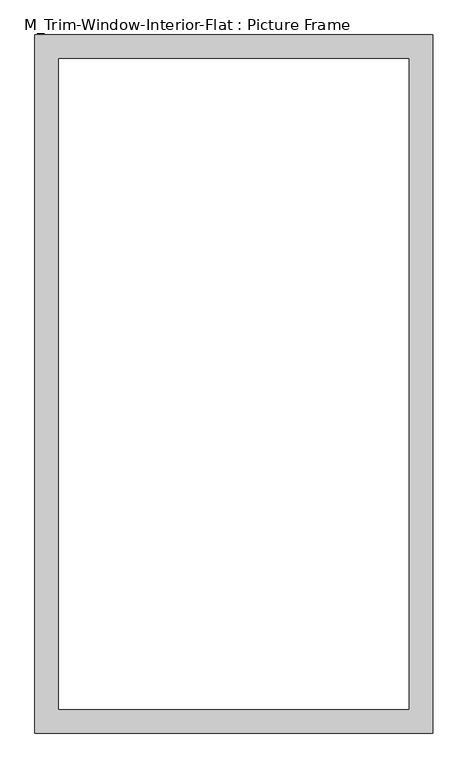
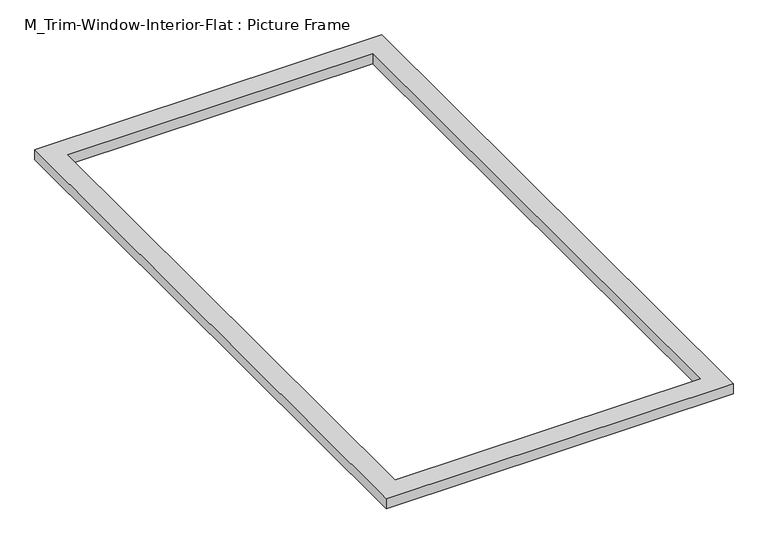
"""IFC4 building model written with IfcOpenShell, lengths in millimetres: proxy geometry, M_Trim-Window-Interior-Flat : Picture Frame."""

import ifcopenshell
import ifcopenshell.guid

model = None  # the IFC model being written
_history = None  # IfcOwnerHistory: only IFC2X3 demands one
_inside = {}  # id of a spatial element -> (the spatial element, [elements in it])
_under = {}  # id of a project, library or spatial element -> (it, [spatial elements below it])
_declared = {}  # id of a project -> (the project, [libraries it declares])
_typed = {}  # id of a type object -> (the type object, [elements of that type])
_made_of = {}  # id of a material, layer set ... -> (it, [elements and type objects made of it])


def new_model(schema):
    """Start an empty IFC model of exactly this schema.

    Asked for "IFC4X3", IfcOpenShell would pick the latest addendum, in which some entities
    have other attributes; the version numbers below select the first issue.
    IFC2X3 requires an IfcOwnerHistory on every rooted entity: one is made here for all.
    """
    global model, _history
    if schema == "IFC4X3":
        model = ifcopenshell.file(schema_version=(4, 3, 0, 0))
    else:
        model = ifcopenshell.file(schema=schema)
    _inside.clear()
    _under.clear()
    _declared.clear()
    _typed.clear()
    _made_of.clear()
    _history = None
    if model.schema == "IFC2X3":
        org = make("IfcOrganization", Name="unknown")
        user = make(
            "IfcPersonAndOrganization",
            ThePerson=make("IfcPerson", FamilyName="unknown"),
            TheOrganization=org,
        )
        app = make(
            "IfcApplication",
            ApplicationDeveloper=org,
            Version="unknown",
            ApplicationFullName="unknown",
            ApplicationIdentifier="unknown",
        )
        _history = make(
            "IfcOwnerHistory",
            OwningUser=user,
            OwningApplication=app,
            ChangeAction="ADDED",
            CreationDate=0,
        )
    return model


def make(cls, **values):
    """One entity of the class cls with the attributes given. An attribute that is None is left unset."""
    return model.create_entity(
        cls, **{name: value for name, value in values.items() if value is not None}
    )


def rooted(cls, **values):
    """An entity with a GlobalId (a new one), such as an element, a storey or a relation."""
    return make(cls, GlobalId=ifcopenshell.guid.new(), OwnerHistory=_history, **values)


def si_unit(unit_type, name, prefix=None):
    """IfcSIUnit, for example si_unit("LENGTHUNIT", "METRE", prefix="MILLI")."""
    return make("IfcSIUnit", UnitType=unit_type, Prefix=prefix, Name=name)


def assignment(units):
    """IfcUnitAssignment: the units of a project."""
    return None if units is None else make("IfcUnitAssignment", Units=units)


def point(xyz):
    """IfcCartesianPoint."""
    return None if xyz is None else make("IfcCartesianPoint", Coordinates=xyz)


def direction(xyz):
    """IfcDirection."""
    return None if xyz is None else make("IfcDirection", DirectionRatios=xyz)


def frame(location, z_axis=None, x_axis=None):
    """IfcAxis2Placement3D, a coordinate frame: its origin and axes. An axis left out is left unset."""
    return make(
        "IfcAxis2Placement3D",
        Location=point(location),
        Axis=direction(z_axis),
        RefDirection=direction(x_axis),
    )


def origin():
    """The frame at (0, 0, 0) with its axes left unset."""
    return frame((0.0, 0.0, 0.0))


def origin_with_axes():
    """The frame at (0, 0, 0) with the z axis (0, 0, 1) and the x axis (1, 0, 0) written out."""
    return frame((0.0, 0.0, 0.0), z_axis=(0.0, 0.0, 1.0), x_axis=(1.0, 0.0, 0.0))


def place(relative_to, where):
    """IfcLocalPlacement: puts the frame where relative to a parent placement (None: the world)."""
    return make(
        "IfcLocalPlacement", PlacementRelTo=relative_to, RelativePlacement=where
    )


def context(
    kind, dimensions, precision=None, world=None, true_north=None, identifier=None
):
    """IfcGeometricRepresentationContext, for example the 3D "Model" context."""
    return make(
        "IfcGeometricRepresentationContext",
        ContextIdentifier=identifier,
        ContextType=kind,
        CoordinateSpaceDimension=dimensions,
        Precision=precision,
        WorldCoordinateSystem=world,
        TrueNorth=true_north,
    )


def project(units=None, contexts=None):
    """IfcProject with its units and contexts."""
    return rooted(
        "IfcProject",
        Name="project",
        RepresentationContexts=contexts,
        UnitsInContext=assignment(units),
    )


def spatial(cls, under=None, at=None, **own):
    """A site, building, storey or space (cls), placed at a placement, below another one or the project."""
    s = rooted(cls, ObjectPlacement=at, **own)
    if under is not None:
        _under.setdefault(under.id(), (under, []))[1].append(s)
    return s


def polyline(points):
    """IfcPolyline through the points."""
    return make("IfcPolyline", Points=[point(p) for p in points])


def outline(outer, holes=None, kind="AREA"):
    """IfcArbitraryClosedProfileDef: a profile drawn as a closed curve; with holes, ...WithVoids."""
    if holes is None:
        return make("IfcArbitraryClosedProfileDef", ProfileType=kind, OuterCurve=outer)
    return make(
        "IfcArbitraryProfileDefWithVoids",
        ProfileType=kind,
        OuterCurve=outer,
        InnerCurves=holes,
    )


def extrude(swept, where, along, depth):
    """IfcExtrudedAreaSolid: the profile swept, set in the frame where, extruded along a direction by depth."""
    return make(
        "IfcExtrudedAreaSolid",
        SweptArea=swept,
        Position=where,
        ExtrudedDirection=direction(along),
        Depth=depth,
    )


def shape(context_of_items, identifier, shape_type, items):
    """IfcShapeRepresentation: the items that make up one representation, for example the "Body"."""
    return make(
        "IfcShapeRepresentation",
        ContextOfItems=context_of_items,
        RepresentationIdentifier=identifier,
        RepresentationType=shape_type,
        Items=items,
    )


def source(mapping_origin, context_of_items, identifier, shape_type, items):
    """IfcRepresentationMap: a shape defined once, which mapped items show again and again."""
    return make(
        "IfcRepresentationMap",
        MappingOrigin=mapping_origin,
        MappedRepresentation=shape(context_of_items, identifier, shape_type, items),
    )


def transform(
    local_origin,
    x_axis=None,
    y_axis=None,
    z_axis=None,
    scale=None,
    scale2=None,
    scale3=None,
    uniform=True,
):
    """IfcCartesianTransformationOperator3D, or its non-uniform kind. x_axis, y_axis, z_axis: its Axis1, 2, 3."""
    if uniform:
        return make(
            "IfcCartesianTransformationOperator3D",
            Axis1=direction(x_axis),
            Axis2=direction(y_axis),
            LocalOrigin=point(local_origin),
            Scale=scale,
            Axis3=direction(z_axis),
        )
    return make(
        "IfcCartesianTransformationOperator3DnonUniform",
        Axis1=direction(x_axis),
        Axis2=direction(y_axis),
        LocalOrigin=point(local_origin),
        Scale=scale,
        Axis3=direction(z_axis),
        Scale2=scale2,
        Scale3=scale3,
    )


def mapped(mapping_source, mapping_target):
    """IfcMappedItem: shows the shape of a source again, moved by a transform."""
    return make(
        "IfcMappedItem", MappingSource=mapping_source, MappingTarget=mapping_target
    )


def made_of(thing, what):
    """Note that an element or type object is made of a material, layer set ...; save() writes the relation."""
    if what is not None:
        _made_of.setdefault(what.id(), (what, []))[1].append(thing)
    return thing


def element(
    cls,
    number,
    at=None,
    inside=None,
    cuts=None,
    type_object=None,
    material=None,
    context=None,
    identifier="Body",
    shape_type=None,
    held_by="IfcProductDefinitionShape",
    body=None,
    shapes=None,
    **own,
):
    """One element of the class cls, such as IfcWall. Its Tag is "e" and its number.

    at: its placement. inside: the storey or other place that contains it. cuts: it is an
    opening in that element (IfcRelVoidsElement). A single representation is given by context,
    identifier, shape_type and body (its items); several are given by shapes. held_by: the class
    of the entity that holds the representations. save() writes the other relations.
    """
    e = rooted(cls, Tag="e%d" % number, ObjectPlacement=at, **own)
    if body is not None:
        shapes = [shape(context, identifier, shape_type, body)]
    if shapes is not None:
        e.Representation = make(held_by, Representations=shapes)
    if inside is not None:
        _inside.setdefault(inside.id(), (inside, []))[1].append(e)
    if cuts is not None:
        rooted(
            "IfcRelVoidsElement", RelatingBuildingElement=cuts, RelatedOpeningElement=e
        )
    if type_object is not None:
        _typed.setdefault(type_object.id(), (type_object, []))[1].append(e)
    return made_of(e, material)


def aggregate(whole, parts):
    """IfcRelAggregates: a whole, such as a stair, and the parts it consists of."""
    return rooted("IfcRelAggregates", RelatingObject=whole, RelatedObjects=parts)


def save(model, path):
    """Write the relations noted so far, then the file.

    IfcRelAggregates (storeys below a building ...), IfcRelContainedInSpatialStructure (elements
    in a storey), IfcRelDefinesByType, IfcRelAssociatesMaterial and IfcRelDeclares: one each for
    every whole, place, type object, material and project.
    """
    for whole, parts in _under.values():
        aggregate(whole, parts)
    for where, things in _inside.values():
        rooted(
            "IfcRelContainedInSpatialStructure",
            RelatedElements=things,
            RelatingStructure=where,
        )
    for kind, things in _typed.values():
        rooted("IfcRelDefinesByType", RelatedObjects=things, RelatingType=kind)
    for what, things in _made_of.values():
        rooted("IfcRelAssociatesMaterial", RelatedObjects=things, RelatingMaterial=what)
    for by, libraries in _declared.values():
        rooted("IfcRelDeclares", RelatingContext=by, RelatedDefinitions=libraries)
    model.write(path)


def m_trim_window_interior_flat_picture_frame_313add5a(model_context):
    return source(origin(), model_context, "Body", "SweptSolid", [
        extrude(outline(polyline([(497.3, 47.3), (497.3, -1697.3), (-497.3, -1697.3), (-497.3, 47.3), (497.3, 47.3)]), holes=[polyline([(437.3, -12.7), (-437.3, -12.7), (-437.3, -1637.3), (437.3, -1637.3), (437.3, -12.7)])]), origin_with_axes(), (0.0, 0.0, 1.0), 30.0),
    ])


if __name__ == "__main__":
    model = new_model("IFC4")
    model_context = context("Model", 3, world=origin())
    ifc_project = project(units=[si_unit("LENGTHUNIT", "METRE", prefix="MILLI")], contexts=[model_context])
    site = spatial("IfcSite", under=ifc_project)
    building = spatial("IfcBuilding", under=site)
    placement = place(None, origin())
    m_trim_window_interior_flat_picture_frame_shape = m_trim_window_interior_flat_picture_frame_313add5a(model_context)
    element("IfcBuildingElementProxy", 1, Name="M_Trim-Window-Interior-Flat : Picture Frame", ObjectType="M_Trim-Window-Interior-Flat : Picture Frame", at=placement, inside=building, context=model_context, shape_type="MappedRepresentation", body=[
        mapped(m_trim_window_interior_flat_picture_frame_shape, transform((0.0, 0.0, 0.0), x_axis=(1.0, 0.0, 0.0), y_axis=(0.0, 1.0, 0.0), z_axis=(0.0, 0.0, 1.0))),
    ])
    save(model, "model.ifc")

# Revit data of these elements
# Type "M_Trim-Window-Interior-Flat : Picture Frame"
#   Trim Thickness_Picture Frame = 30 mm
#   Trim Width = 60 mm
#   Trim Thickness_with Sill = 20 mm
#   Sill Thickness = 30 mm
#   Opening Width [instance default] = 600 mm
#   Opening Height [instance default] = 900 mm
#   Default Elevation = 1200 mm
#   Sill = no
#   Picture Frame = yes
#   Trim Material [instance default] = none
# Element 1 (IfcBuildingElementProxy, "M_Trim-Window-Interior-Flat : Picture Frame")
#   Opening Width = 900 mm
#   Opening Height = 1650 mm
#   Trim Material = Wood - Stained
#   Materials on its faces: "Wood - Stained"
# Materials
#   "Wood - Stained": class "Wood", colour RGB 173 132 96, transparency 0, Cost = 0
